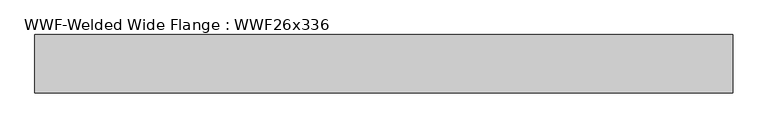
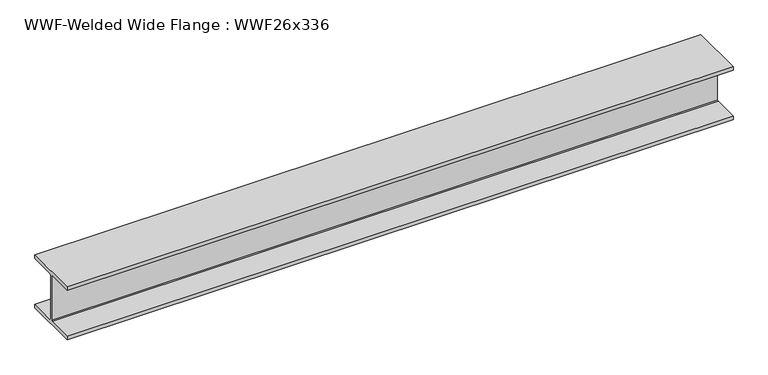
"""IFC4 building model written with IfcOpenShell, lengths in millimetres: beam geometry, WWF-Welded Wide Flange : WWF26x336."""

import ifcopenshell
import ifcopenshell.guid

model = None  # the IFC model being written
_history = None  # IfcOwnerHistory: only IFC2X3 demands one
_inside = {}  # id of a spatial element -> (the spatial element, [elements in it])
_under = {}  # id of a project, library or spatial element -> (it, [spatial elements below it])
_declared = {}  # id of a project -> (the project, [libraries it declares])
_typed = {}  # id of a type object -> (the type object, [elements of that type])
_made_of = {}  # id of a material, layer set ... -> (it, [elements and type objects made of it])


def new_model(schema):
    """Start an empty IFC model of exactly this schema.

    Asked for "IFC4X3", IfcOpenShell would pick the latest addendum, in which some entities
    have other attributes; the version numbers below select the first issue.
    IFC2X3 requires an IfcOwnerHistory on every rooted entity: one is made here for all.
    """
    global model, _history
    if schema == "IFC4X3":
        model = ifcopenshell.file(schema_version=(4, 3, 0, 0))
    else:
        model = ifcopenshell.file(schema=schema)
    _inside.clear()
    _under.clear()
    _declared.clear()
    _typed.clear()
    _made_of.clear()
    _history = None
    if model.schema == "IFC2X3":
        org = make("IfcOrganization", Name="unknown")
        user = make(
            "IfcPersonAndOrganization",
            ThePerson=make("IfcPerson", FamilyName="unknown"),
            TheOrganization=org,
        )
        app = make(
            "IfcApplication",
            ApplicationDeveloper=org,
            Version="unknown",
            ApplicationFullName="unknown",
            ApplicationIdentifier="unknown",
        )
        _history = make(
            "IfcOwnerHistory",
            OwningUser=user,
            OwningApplication=app,
            ChangeAction="ADDED",
            CreationDate=0,
        )
    return model


def make(cls, **values):
    """One entity of the class cls with the attributes given. An attribute that is None is left unset."""
    return model.create_entity(
        cls, **{name: value for name, value in values.items() if value is not None}
    )


def rooted(cls, **values):
    """An entity with a GlobalId (a new one), such as an element, a storey or a relation."""
    return make(cls, GlobalId=ifcopenshell.guid.new(), OwnerHistory=_history, **values)


def si_unit(unit_type, name, prefix=None):
    """IfcSIUnit, for example si_unit("LENGTHUNIT", "METRE", prefix="MILLI")."""
    return make("IfcSIUnit", UnitType=unit_type, Prefix=prefix, Name=name)


def assignment(units):
    """IfcUnitAssignment: the units of a project."""
    return None if units is None else make("IfcUnitAssignment", Units=units)


def point(xyz):
    """IfcCartesianPoint."""
    return None if xyz is None else make("IfcCartesianPoint", Coordinates=xyz)


def direction(xyz):
    """IfcDirection."""
    return None if xyz is None else make("IfcDirection", DirectionRatios=xyz)


def frame(location, z_axis=None, x_axis=None):
    """IfcAxis2Placement3D, a coordinate frame: its origin and axes. An axis left out is left unset."""
    return make(
        "IfcAxis2Placement3D",
        Location=point(location),
        Axis=direction(z_axis),
        RefDirection=direction(x_axis),
    )


def origin():
    """The frame at (0, 0, 0) with its axes left unset."""
    return frame((0.0, 0.0, 0.0))


def place(relative_to, where):
    """IfcLocalPlacement: puts the frame where relative to a parent placement (None: the world)."""
    return make(
        "IfcLocalPlacement", PlacementRelTo=relative_to, RelativePlacement=where
    )


def context(
    kind, dimensions, precision=None, world=None, true_north=None, identifier=None
):
    """IfcGeometricRepresentationContext, for example the 3D "Model" context."""
    return make(
        "IfcGeometricRepresentationContext",
        ContextIdentifier=identifier,
        ContextType=kind,
        CoordinateSpaceDimension=dimensions,
        Precision=precision,
        WorldCoordinateSystem=world,
        TrueNorth=true_north,
    )


def project(units=None, contexts=None):
    """IfcProject with its units and contexts."""
    return rooted(
        "IfcProject",
        Name="project",
        RepresentationContexts=contexts,
        UnitsInContext=assignment(units),
    )


def spatial(cls, under=None, at=None, **own):
    """A site, building, storey or space (cls), placed at a placement, below another one or the project."""
    s = rooted(cls, ObjectPlacement=at, **own)
    if under is not None:
        _under.setdefault(under.id(), (under, []))[1].append(s)
    return s


def polyline(points):
    """IfcPolyline through the points."""
    return make("IfcPolyline", Points=[point(p) for p in points])


def outline(outer, holes=None, kind="AREA"):
    """IfcArbitraryClosedProfileDef: a profile drawn as a closed curve; with holes, ...WithVoids."""
    if holes is None:
        return make("IfcArbitraryClosedProfileDef", ProfileType=kind, OuterCurve=outer)
    return make(
        "IfcArbitraryProfileDefWithVoids",
        ProfileType=kind,
        OuterCurve=outer,
        InnerCurves=holes,
    )


def extrude(swept, where, along, depth):
    """IfcExtrudedAreaSolid: the profile swept, set in the frame where, extruded along a direction by depth."""
    return make(
        "IfcExtrudedAreaSolid",
        SweptArea=swept,
        Position=where,
        ExtrudedDirection=direction(along),
        Depth=depth,
    )


def shape(context_of_items, identifier, shape_type, items):
    """IfcShapeRepresentation: the items that make up one representation, for example the "Body"."""
    return make(
        "IfcShapeRepresentation",
        ContextOfItems=context_of_items,
        RepresentationIdentifier=identifier,
        RepresentationType=shape_type,
        Items=items,
    )


def source(mapping_origin, context_of_items, identifier, shape_type, items):
    """IfcRepresentationMap: a shape defined once, which mapped items show again and again."""
    return make(
        "IfcRepresentationMap",
        MappingOrigin=mapping_origin,
        MappedRepresentation=shape(context_of_items, identifier, shape_type, items),
    )


def transform(
    local_origin,
    x_axis=None,
    y_axis=None,
    z_axis=None,
    scale=None,
    scale2=None,
    scale3=None,
    uniform=True,
):
    """IfcCartesianTransformationOperator3D, or its non-uniform kind. x_axis, y_axis, z_axis: its Axis1, 2, 3."""
    if uniform:
        return make(
            "IfcCartesianTransformationOperator3D",
            Axis1=direction(x_axis),
            Axis2=direction(y_axis),
            LocalOrigin=point(local_origin),
            Scale=scale,
            Axis3=direction(z_axis),
        )
    return make(
        "IfcCartesianTransformationOperator3DnonUniform",
        Axis1=direction(x_axis),
        Axis2=direction(y_axis),
        LocalOrigin=point(local_origin),
        Scale=scale,
        Axis3=direction(z_axis),
        Scale2=scale2,
        Scale3=scale3,
    )


def mapped(mapping_source, mapping_target):
    """IfcMappedItem: shows the shape of a source again, moved by a transform."""
    return make(
        "IfcMappedItem", MappingSource=mapping_source, MappingTarget=mapping_target
    )


def made_of(thing, what):
    """Note that an element or type object is made of a material, layer set ...; save() writes the relation."""
    if what is not None:
        _made_of.setdefault(what.id(), (what, []))[1].append(thing)
    return thing


def element(
    cls,
    number,
    at=None,
    inside=None,
    cuts=None,
    type_object=None,
    material=None,
    context=None,
    identifier="Body",
    shape_type=None,
    held_by="IfcProductDefinitionShape",
    body=None,
    shapes=None,
    **own,
):
    """One element of the class cls, such as IfcWall. Its Tag is "e" and its number.

    at: its placement. inside: the storey or other place that contains it. cuts: it is an
    opening in that element (IfcRelVoidsElement). A single representation is given by context,
    identifier, shape_type and body (its items); several are given by shapes. held_by: the class
    of the entity that holds the representations. save() writes the other relations.
    """
    e = rooted(cls, Tag="e%d" % number, ObjectPlacement=at, **own)
    if body is not None:
        shapes = [shape(context, identifier, shape_type, body)]
    if shapes is not None:
        e.Representation = make(held_by, Representations=shapes)
    if inside is not None:
        _inside.setdefault(inside.id(), (inside, []))[1].append(e)
    if cuts is not None:
        rooted(
            "IfcRelVoidsElement", RelatingBuildingElement=cuts, RelatedOpeningElement=e
        )
    if type_object is not None:
        _typed.setdefault(type_object.id(), (type_object, []))[1].append(e)
    return made_of(e, material)


def aggregate(whole, parts):
    """IfcRelAggregates: a whole, such as a stair, and the parts it consists of."""
    return rooted("IfcRelAggregates", RelatingObject=whole, RelatedObjects=parts)


def save(model, path):
    """Write the relations noted so far, then the file.

    IfcRelAggregates (storeys below a building ...), IfcRelContainedInSpatialStructure (elements
    in a storey), IfcRelDefinesByType, IfcRelAssociatesMaterial and IfcRelDeclares: one each for
    every whole, place, type object, material and project.
    """
    for whole, parts in _under.values():
        aggregate(whole, parts)
    for where, things in _inside.values():
        rooted(
            "IfcRelContainedInSpatialStructure",
            RelatedElements=things,
            RelatingStructure=where,
        )
    for kind, things in _typed.values():
        rooted("IfcRelDefinesByType", RelatedObjects=things, RelatingType=kind)
    for what, things in _made_of.values():
        rooted("IfcRelAssociatesMaterial", RelatedObjects=things, RelatingMaterial=what)
    for by, libraries in _declared.values():
        rooted("IfcRelDeclares", RelatingContext=by, RelatedDefinitions=libraries)
    model.write(path)


def wwf_welded_wide_flange_wwf26x336_54fb23f7(model_context):
    return source(origin(), model_context, "Body", "SweptSolid", [
        extrude(outline(polyline([(324.993, -284.988), (324.993, -324.993), (-324.993, -324.993), (-324.993, -284.988), (-20.6375, -284.988), (-9.9949, -274.3454), (-9.9949, 274.3454), (-20.6375, 284.988), (-324.993, 284.988), (-324.993, 324.993), (324.993, 324.993), (324.993, 284.988), (20.6375, 284.988), (9.9949, 274.3454), (9.9949, -274.3454), (20.6375, -284.988), (324.993, -284.988)])), frame((-3934.8877112, 0.0, 0.0), z_axis=(1.0, 0.0, 0.0), x_axis=(0.0, 1.0, 0.0)), (0.0, 0.0, 1.0), 7762.6459669),
    ])


if __name__ == "__main__":
    model = new_model("IFC4")
    model_context = context("Model", 3, world=origin())
    ifc_project = project(units=[si_unit("LENGTHUNIT", "METRE", prefix="MILLI")], contexts=[model_context])
    site = spatial("IfcSite", under=ifc_project)
    building = spatial("IfcBuilding", under=site)
    placement = place(None, origin())
    wwf_welded_wide_flange_wwf26x336_shape = wwf_welded_wide_flange_wwf26x336_54fb23f7(model_context)
    element("IfcBeam", 1, ObjectType="WWF-Welded Wide Flange : WWF26x336", at=placement, inside=building, context=model_context, shape_type="MappedRepresentation", body=[
        mapped(wwf_welded_wide_flange_wwf26x336_shape, transform((0.0, 0.0, 0.0), x_axis=(1.0, 0.0, 0.0), y_axis=(0.0, 1.0, 0.0), z_axis=(0.0, 0.0, 1.0))),
    ])
    save(model, "model.ifc")

# Revit data of these elements
# Type "WWF-Welded Wide Flange : WWF26x336"
#   Assembly Code = "B10"
#   Nominal d = "12"
#   W = 336
#   Length [instance default] = 1524 mm
#   bf = 649.986 mm
#   d = 649.986 mm
#   k = 20.638 mm
#   tf = 40.005 mm
#   tw = 19.99 mm
#   A = 0.0635483 m²
#   Structural Material [instance default] = Steel ASTM A572
# Element 1 (IfcBeam, "WWF-Welded Wide Flange : WWF26x336")
#   Structural Material = Metal - Steel 43-275
#   Materials on its faces: "Metal - Steel 43-275"
# Materials
#   "Steel ASTM A572": class "Metal", colour RGB 247 247 247, transparency 0, Description = "Structural steel, high strength low alloy, ASTM - A572 - 50", Cost = 0
#   "Metal - Steel 43-275": class "Metal", colour RGB 247 247 247, transparency 0, Cost = 0
